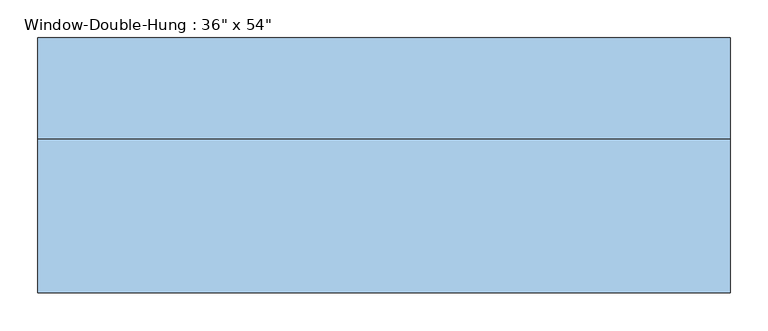
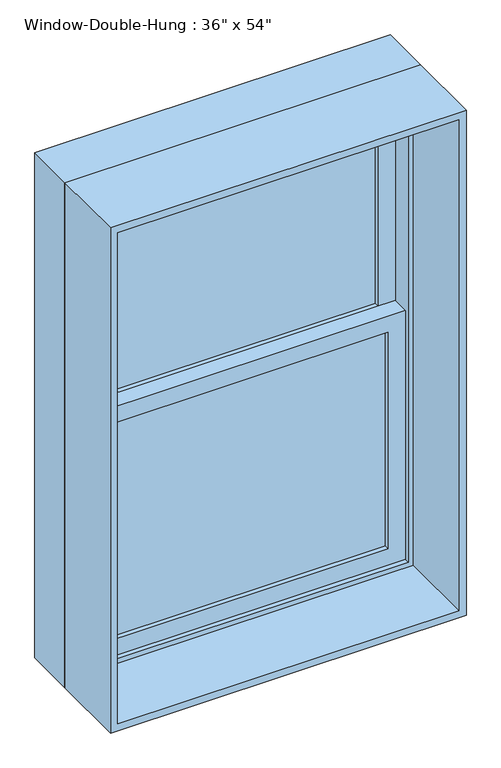
"""IFC4 building model written with IfcOpenShell, lengths in millimetres: window geometry."""

from ifc_helpers import new_model, si_unit, frame, origin, place, context, project, spatial, polyline, outline, extrude, source, transform, mapped, element, save


def window_5aee1ffa(model_context):
    return source(origin(), model_context, "Body", "SweptSolid", [
        extrude(outline(polyline([(381.0, 88.9), (381.0, 82.55), (-381.0, 82.55), (-381.0, 88.9), (381.0, 88.9)])), frame((0.0, 0.0, 990.6), z_axis=(0.0, 0.0, 1.0), x_axis=(1.0, 0.0, 0.0)), (0.0, 0.0, 1.0), 587.375),
        extrude(outline(polyline([(-381.0, 76.2), (381.0, 76.2), (381.0, 69.85), (-381.0, 69.85), (-381.0, 76.2)])), frame((0.0, 0.0, 990.6), z_axis=(0.0, 0.0, 1.0), x_axis=(1.0, 0.0, 0.0)), (0.0, 0.0, 1.0), 587.375),
        extrude(outline(polyline([(381.0, 133.35), (381.0, 127.0), (-381.0, 127.0), (-381.0, 133.35), (381.0, 133.35)])), frame((0.0, 0.0, 1622.425), z_axis=(0.0, 0.0, 1.0), x_axis=(1.0, 0.0, 0.0)), (0.0, 0.0, 1.0), 587.375),
        extrude(outline(polyline([(-381.0, 120.65), (381.0, 120.65), (381.0, 114.3), (-381.0, 114.3), (-381.0, 120.65)])), frame((0.0, 0.0, 1622.425), z_axis=(0.0, 0.0, 1.0), x_axis=(1.0, 0.0, 0.0)), (0.0, 0.0, 1.0), 587.375),
        extrude(outline(polyline([(1622.425, -425.45), (946.15, -425.45), (946.15, 425.45), (1622.425, 425.45), (1622.425, -425.45)]), holes=[polyline([(1577.975, 381.0), (990.6, 381.0), (990.6, -381.0), (1577.975, -381.0), (1577.975, 381.0)])]), frame((0.0, 57.15, 0.0), z_axis=(0.0, 1.0, 0.0), x_axis=(0.0, 0.0, 1.0)), (0.0, 0.0, 1.0), 44.45),
        extrude(outline(polyline([(2254.25, -425.45), (1577.975, -425.45), (1577.975, 425.45), (2254.25, 425.45), (2254.25, -425.45)]), holes=[polyline([(2209.8, 381.0), (1622.425, 381.0), (1622.425, -381.0), (2209.8, -381.0), (2209.8, 381.0)])]), frame((0.0, 101.6, 0.0), z_axis=(0.0, 1.0, 0.0), x_axis=(0.0, 0.0, 1.0)), (0.0, 0.0, 1.0), 44.45),
        extrude(outline(polyline([(2286.0, -457.2), (914.4, -457.2), (914.4, 457.2), (2286.0, 457.2), (2286.0, -457.2)]), holes=[polyline([(2254.25, 425.45), (946.15, 425.45), (946.15, -425.45), (2254.25, -425.45), (2254.25, 425.45)])]), frame((0.0, 44.45, 0.0), z_axis=(0.0, 1.0, 0.0), x_axis=(0.0, 0.0, 1.0)), (0.0, 0.0, 1.0), 133.35),
        extrude(outline(polyline([(2286.0, 457.2), (2286.0, -457.2), (914.4, -457.2), (914.4, 457.2), (2286.0, 457.2)]), holes=[polyline([(2266.95, 438.15), (933.45, 438.15), (933.45, -438.15), (2266.95, -438.15), (2266.95, 438.15)])]), frame((0.0, -158.75, 0.0), z_axis=(0.0, 1.0, 0.0), x_axis=(0.0, 0.0, 1.0)), (0.0, 0.0, 1.0), 203.2),
    ])


if __name__ == "__main__":
    model = new_model("IFC4")
    model_context = context("Model", 3, world=origin())
    ifc_project = project(units=[si_unit("LENGTHUNIT", "METRE", prefix="MILLI")], contexts=[model_context])
    site = spatial("IfcSite", under=ifc_project)
    building = spatial("IfcBuilding", under=site)
    placement = place(None, origin())
    window_shape = window_5aee1ffa(model_context)
    element("IfcWindow", 1, ObjectType="Window-Double-Hung : 36\" x 54\"", at=placement, inside=building, context=model_context, shape_type="MappedRepresentation", body=[
        mapped(window_shape, transform((0.0, 0.0, 0.0), x_axis=(1.0, 0.0, 0.0), y_axis=(0.0, 1.0, 0.0), z_axis=(0.0, 0.0, 1.0))),
    ])
    save(model, "model.ifc")

# Revit data of these elements
# Type "Window-Double-Hung : 36\" x 54\""
#   Type Mark = "18"
#   Fire Rating = "0.5h"
#   Construction Type Id = "DG-DR"
#   Assembly Code = "B2020100"
#   Analytic Construction = "Double glazing - domestic"
#   Wall Thickness [instance default] = 0' - 6"
#   Window Inset [instance default] = 0' - 0"
#   Visual Light Transmittance = 0.81
#   Thermal Resistance (R) = 1.8146 (h·ft²·°F)/BTU
#   Solar Heat Gain Coefficient = 0.76
#   Muntin Width = 2' - 6"
#   Muntin Height = 1' - 11 1/8"
#   Interior Wall Closure [instance default] = 0' - 1 1/2"
#   Rough Width = 3' - 0 1/2"
#   Rough Height = 4' - 6 1/2"
#   Frame Extension [instance default] = 0' - 1 1/4"
#   Exterior Wall Closure [instance default] = 0' - 0 1/2"
#   Extension Jamb [instance default] = 0' - 1 1/2"
#   Heat Transfer Coefficient (U) = 0.5511 BTU/(h·ft²·°F)
#   Height = 4' - 6"
#   Width = 3' - 0"
#   Top Muntin Visibility = yes
#   Indicator Visibility [instance default] = yes
#   Extension Jamb Visibility [instance default] = yes
#   Interior Trim Visibility [instance default] = yes
#   Exterior Trim Visibility [instance default] = yes
#   Define Thermal Properties by = 1
#   Bottom Muntin Visibility = yes
#   Muntin Pattern = Muntin Pattern_2x2 : Muntin Pattern_2x2
#   Interior Trim Material = Maple - Semigloss(Rotated)
#   Interior Trim = Trim-Window-Interior-Flat : Picture Frame
#   Exterior Trim Material = Clad - White
#   Exterior Trim = Trim-Window-Exterior-Flat : with Sill
#   Glass Panel Material = Glass, Clear Glazing
#   Exterior Frame Material = Clad - White
#   Interior Frame Material = Maple - Semigloss(Rotated)
#   Wall Closure = (empty or 0)
# Element 1 (IfcWindow, "Window-Double-Hung : 36\" x 54\"")
#   Wall Thickness = 1' - 0 1/2"
#   Extension Jamb = 0' - 8"
#   Materials on its faces: "Maple - Semigloss(Rotated)", "Glass, Clear Glazing", "Clad - White"
# Materials
#   "Maple - Semigloss(Rotated)": class "Wood", colour RGB 196 161 118, transparency 0, Description = "Acer Saccharum", Cost = 0
#   "Clad - White": class "Wood", colour RGB 245 245 243, transparency 0, Cost = 0
#   "Glass, Clear Glazing": class "Glass", colour RGB 245 245 243, transparency 1, Description = "Clear glazing", Cost = 0
